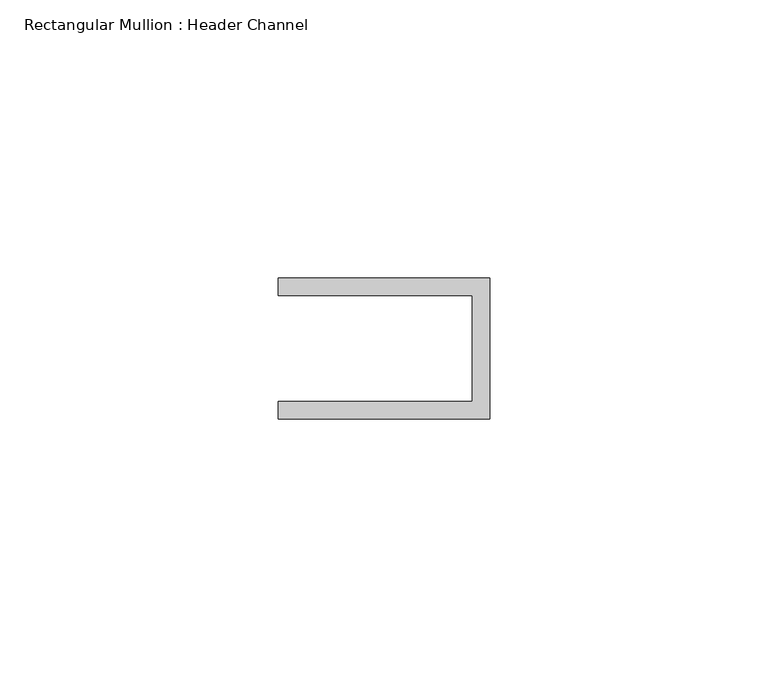
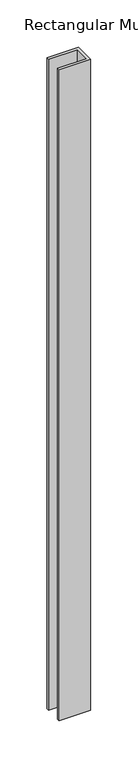
"""IFC4 building model written with IfcOpenShell, lengths in millimetres: member geometry, Rectangular Mullion : Header Channel."""

from ifc_helpers import new_model, si_unit, frame, origin, place, context, project, spatial, polyline, outline, extrude, source, transform, mapped, element, save


def rectangular_mullion_header_channel_ba5daf2f(model_context):
    return source(origin(), model_context, "Body", "SweptSolid", [
        extrude(outline(polyline([(0.0, -12.7), (-38.1, -12.7), (-38.1, -9.525), (-3.175, -9.525), (-3.175, 9.525), (-38.1, 9.525), (-38.1, 12.7), (0.0, 12.7), (0.0, -12.7)])), frame((0.0, 0.0, -838.2000002), z_axis=(0.0, 0.0, 1.0), x_axis=(1.0, 0.0, 0.0)), (0.0, 0.0, 1.0), 838.2000002),
    ])


if __name__ == "__main__":
    model = new_model("IFC4")
    model_context = context("Model", 3, world=origin())
    ifc_project = project(units=[si_unit("LENGTHUNIT", "METRE", prefix="MILLI")], contexts=[model_context])
    site = spatial("IfcSite", under=ifc_project)
    building = spatial("IfcBuilding", under=site)
    placement = place(None, origin())
    rectangular_mullion_header_channel_shape = rectangular_mullion_header_channel_ba5daf2f(model_context)
    element("IfcMember", 1, ObjectType="Rectangular Mullion : Header Channel", at=placement, inside=building, context=model_context, shape_type="MappedRepresentation", body=[
        mapped(rectangular_mullion_header_channel_shape, transform((0.0, 0.0, 0.0), x_axis=(1.0, 0.0, 0.0), y_axis=(0.0, 1.0, 0.0), z_axis=(0.0, 0.0, 1.0))),
    ])
    save(model, "model.ifc")

# Revit data of these elements
# Type "Rectangular Mullion : Header Channel"
#   built-in parameter 1007322 = 0.0833333 (stored number, unit not read)
#   built-in parameter 1007321 = -0.03125 (stored number, unit not read)
#   built-in parameter 1007320 = 0.0416667 (stored number, unit not read)
# Element 1 (IfcMember, "Rectangular Mullion : Header Channel")
#   Materials on its faces: "ALUM"
# Materials
#   "ALUM": class "Generic", colour RGB 157 157 157, transparency 0, Cost = 0
